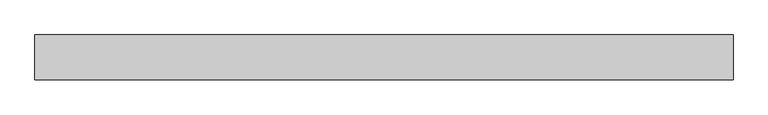
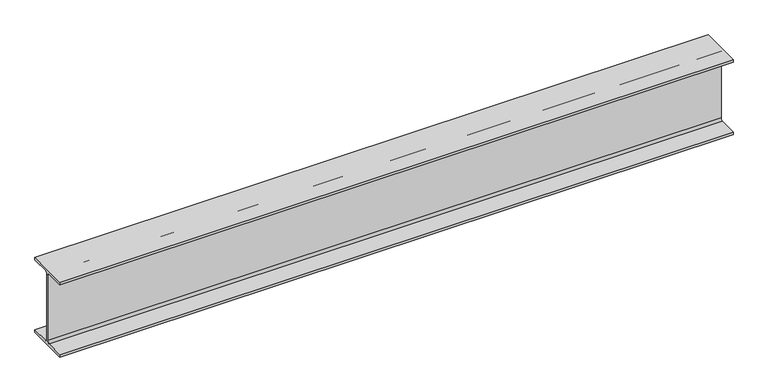
"""IFC4 building model written with IfcOpenShell, lengths in millimetres: beam geometry, Steel Beam_H-KSD3502 : H_SB_ASB_H-194x150x6x9."""

import ifcopenshell
import ifcopenshell.guid

model = None  # the IFC model being written
_history = None  # IfcOwnerHistory: only IFC2X3 demands one
_inside = {}  # id of a spatial element -> (the spatial element, [elements in it])
_under = {}  # id of a project, library or spatial element -> (it, [spatial elements below it])
_declared = {}  # id of a project -> (the project, [libraries it declares])
_typed = {}  # id of a type object -> (the type object, [elements of that type])
_made_of = {}  # id of a material, layer set ... -> (it, [elements and type objects made of it])


def new_model(schema):
    """Start an empty IFC model of exactly this schema.

    Asked for "IFC4X3", IfcOpenShell would pick the latest addendum, in which some entities
    have other attributes; the version numbers below select the first issue.
    IFC2X3 requires an IfcOwnerHistory on every rooted entity: one is made here for all.
    """
    global model, _history
    if schema == "IFC4X3":
        model = ifcopenshell.file(schema_version=(4, 3, 0, 0))
    else:
        model = ifcopenshell.file(schema=schema)
    _inside.clear()
    _under.clear()
    _declared.clear()
    _typed.clear()
    _made_of.clear()
    _history = None
    if model.schema == "IFC2X3":
        org = make("IfcOrganization", Name="unknown")
        user = make(
            "IfcPersonAndOrganization",
            ThePerson=make("IfcPerson", FamilyName="unknown"),
            TheOrganization=org,
        )
        app = make(
            "IfcApplication",
            ApplicationDeveloper=org,
            Version="unknown",
            ApplicationFullName="unknown",
            ApplicationIdentifier="unknown",
        )
        _history = make(
            "IfcOwnerHistory",
            OwningUser=user,
            OwningApplication=app,
            ChangeAction="ADDED",
            CreationDate=0,
        )
    return model


def make(cls, **values):
    """One entity of the class cls with the attributes given. An attribute that is None is left unset."""
    return model.create_entity(
        cls, **{name: value for name, value in values.items() if value is not None}
    )


def rooted(cls, **values):
    """An entity with a GlobalId (a new one), such as an element, a storey or a relation."""
    return make(cls, GlobalId=ifcopenshell.guid.new(), OwnerHistory=_history, **values)


def si_unit(unit_type, name, prefix=None):
    """IfcSIUnit, for example si_unit("LENGTHUNIT", "METRE", prefix="MILLI")."""
    return make("IfcSIUnit", UnitType=unit_type, Prefix=prefix, Name=name)


def assignment(units):
    """IfcUnitAssignment: the units of a project."""
    return None if units is None else make("IfcUnitAssignment", Units=units)


def point(xyz):
    """IfcCartesianPoint."""
    return None if xyz is None else make("IfcCartesianPoint", Coordinates=xyz)


def direction(xyz):
    """IfcDirection."""
    return None if xyz is None else make("IfcDirection", DirectionRatios=xyz)


def frame(location, z_axis=None, x_axis=None):
    """IfcAxis2Placement3D, a coordinate frame: its origin and axes. An axis left out is left unset."""
    return make(
        "IfcAxis2Placement3D",
        Location=point(location),
        Axis=direction(z_axis),
        RefDirection=direction(x_axis),
    )


def frame_2d(location, x_axis=None):
    """IfcAxis2Placement2D, a coordinate frame in the plane: its origin and x axis."""
    return make(
        "IfcAxis2Placement2D", Location=point(location), RefDirection=direction(x_axis)
    )


def origin():
    """The frame at (0, 0, 0) with its axes left unset."""
    return frame((0.0, 0.0, 0.0))


def place(relative_to, where):
    """IfcLocalPlacement: puts the frame where relative to a parent placement (None: the world)."""
    return make(
        "IfcLocalPlacement", PlacementRelTo=relative_to, RelativePlacement=where
    )


def context(
    kind, dimensions, precision=None, world=None, true_north=None, identifier=None
):
    """IfcGeometricRepresentationContext, for example the 3D "Model" context."""
    return make(
        "IfcGeometricRepresentationContext",
        ContextIdentifier=identifier,
        ContextType=kind,
        CoordinateSpaceDimension=dimensions,
        Precision=precision,
        WorldCoordinateSystem=world,
        TrueNorth=true_north,
    )


def project(units=None, contexts=None):
    """IfcProject with its units and contexts."""
    return rooted(
        "IfcProject",
        Name="project",
        RepresentationContexts=contexts,
        UnitsInContext=assignment(units),
    )


def spatial(cls, under=None, at=None, **own):
    """A site, building, storey or space (cls), placed at a placement, below another one or the project."""
    s = rooted(cls, ObjectPlacement=at, **own)
    if under is not None:
        _under.setdefault(under.id(), (under, []))[1].append(s)
    return s


def polyline(points):
    """IfcPolyline through the points."""
    return make("IfcPolyline", Points=[point(p) for p in points])


def circle_curve(where, radius):
    """IfcCircle in the frame where."""
    return make("IfcCircle", Position=where, Radius=radius)


def trimmed(basis, trim1, trim2, sense, master):
    """IfcTrimmedCurve: the piece of a basis curve between two trims."""
    return make(
        "IfcTrimmedCurve",
        BasisCurve=basis,
        Trim1=trim1,
        Trim2=trim2,
        SenseAgreement=sense,
        MasterRepresentation=master,
    )


def segment(curve, same_sense, transition):
    """IfcCompositeCurveSegment."""
    return make(
        "IfcCompositeCurveSegment",
        Transition=transition,
        SameSense=same_sense,
        ParentCurve=curve,
    )


def composite_curve(segments, self_intersect=None):
    """IfcCompositeCurve: segments joined end to end."""
    return make("IfcCompositeCurve", Segments=segments, SelfIntersect=self_intersect)


def outline(outer, holes=None, kind="AREA"):
    """IfcArbitraryClosedProfileDef: a profile drawn as a closed curve; with holes, ...WithVoids."""
    if holes is None:
        return make("IfcArbitraryClosedProfileDef", ProfileType=kind, OuterCurve=outer)
    return make(
        "IfcArbitraryProfileDefWithVoids",
        ProfileType=kind,
        OuterCurve=outer,
        InnerCurves=holes,
    )


def extrude(swept, where, along, depth):
    """IfcExtrudedAreaSolid: the profile swept, set in the frame where, extruded along a direction by depth."""
    return make(
        "IfcExtrudedAreaSolid",
        SweptArea=swept,
        Position=where,
        ExtrudedDirection=direction(along),
        Depth=depth,
    )


def shape(context_of_items, identifier, shape_type, items):
    """IfcShapeRepresentation: the items that make up one representation, for example the "Body"."""
    return make(
        "IfcShapeRepresentation",
        ContextOfItems=context_of_items,
        RepresentationIdentifier=identifier,
        RepresentationType=shape_type,
        Items=items,
    )


def source(mapping_origin, context_of_items, identifier, shape_type, items):
    """IfcRepresentationMap: a shape defined once, which mapped items show again and again."""
    return make(
        "IfcRepresentationMap",
        MappingOrigin=mapping_origin,
        MappedRepresentation=shape(context_of_items, identifier, shape_type, items),
    )


def transform(
    local_origin,
    x_axis=None,
    y_axis=None,
    z_axis=None,
    scale=None,
    scale2=None,
    scale3=None,
    uniform=True,
):
    """IfcCartesianTransformationOperator3D, or its non-uniform kind. x_axis, y_axis, z_axis: its Axis1, 2, 3."""
    if uniform:
        return make(
            "IfcCartesianTransformationOperator3D",
            Axis1=direction(x_axis),
            Axis2=direction(y_axis),
            LocalOrigin=point(local_origin),
            Scale=scale,
            Axis3=direction(z_axis),
        )
    return make(
        "IfcCartesianTransformationOperator3DnonUniform",
        Axis1=direction(x_axis),
        Axis2=direction(y_axis),
        LocalOrigin=point(local_origin),
        Scale=scale,
        Axis3=direction(z_axis),
        Scale2=scale2,
        Scale3=scale3,
    )


def mapped(mapping_source, mapping_target):
    """IfcMappedItem: shows the shape of a source again, moved by a transform."""
    return make(
        "IfcMappedItem", MappingSource=mapping_source, MappingTarget=mapping_target
    )


def made_of(thing, what):
    """Note that an element or type object is made of a material, layer set ...; save() writes the relation."""
    if what is not None:
        _made_of.setdefault(what.id(), (what, []))[1].append(thing)
    return thing


def element(
    cls,
    number,
    at=None,
    inside=None,
    cuts=None,
    type_object=None,
    material=None,
    context=None,
    identifier="Body",
    shape_type=None,
    held_by="IfcProductDefinitionShape",
    body=None,
    shapes=None,
    **own,
):
    """One element of the class cls, such as IfcWall. Its Tag is "e" and its number.

    at: its placement. inside: the storey or other place that contains it. cuts: it is an
    opening in that element (IfcRelVoidsElement). A single representation is given by context,
    identifier, shape_type and body (its items); several are given by shapes. held_by: the class
    of the entity that holds the representations. save() writes the other relations.
    """
    e = rooted(cls, Tag="e%d" % number, ObjectPlacement=at, **own)
    if body is not None:
        shapes = [shape(context, identifier, shape_type, body)]
    if shapes is not None:
        e.Representation = make(held_by, Representations=shapes)
    if inside is not None:
        _inside.setdefault(inside.id(), (inside, []))[1].append(e)
    if cuts is not None:
        rooted(
            "IfcRelVoidsElement", RelatingBuildingElement=cuts, RelatedOpeningElement=e
        )
    if type_object is not None:
        _typed.setdefault(type_object.id(), (type_object, []))[1].append(e)
    return made_of(e, material)


def aggregate(whole, parts):
    """IfcRelAggregates: a whole, such as a stair, and the parts it consists of."""
    return rooted("IfcRelAggregates", RelatingObject=whole, RelatedObjects=parts)


def save(model, path):
    """Write the relations noted so far, then the file.

    IfcRelAggregates (storeys below a building ...), IfcRelContainedInSpatialStructure (elements
    in a storey), IfcRelDefinesByType, IfcRelAssociatesMaterial and IfcRelDeclares: one each for
    every whole, place, type object, material and project.
    """
    for whole, parts in _under.values():
        aggregate(whole, parts)
    for where, things in _inside.values():
        rooted(
            "IfcRelContainedInSpatialStructure",
            RelatedElements=things,
            RelatingStructure=where,
        )
    for kind, things in _typed.values():
        rooted("IfcRelDefinesByType", RelatedObjects=things, RelatingType=kind)
    for what, things in _made_of.values():
        rooted("IfcRelAssociatesMaterial", RelatedObjects=things, RelatingMaterial=what)
    for by, libraries in _declared.values():
        rooted("IfcRelDeclares", RelatingContext=by, RelatedDefinitions=libraries)
    model.write(path)


def beam_c1192738(model_context):
    return source(origin(), model_context, "Body", "SweptSolid", [
        extrude(outline(composite_curve([segment(polyline([(82.5, -141.5), (82.5, -151.7), (-82.5, -151.7), (-82.5, -141.5), (-11.9, -141.5)]), True, "CONTINUOUS"), segment(trimmed(circle_curve(frame_2d((-11.9, -132.6)), 8.9), [point((-11.9, -141.5))], [point((-3.0, -132.6))], True, "CARTESIAN"), True, "CONTINUOUS"), segment(polyline([(-3.0, -132.6), (-3.0, 132.6)]), True, "CONTINUOUS"), segment(trimmed(circle_curve(frame_2d((-11.9, 132.6)), 8.9), [point((-3.0, 132.6))], [point((-11.9, 141.5))], True, "CARTESIAN"), True, "CONTINUOUS"), segment(polyline([(-11.9, 141.5), (-82.5, 141.5), (-82.5, 151.7), (82.5, 151.7), (82.5, 141.5), (11.9, 141.5)]), True, "CONTINUOUS"), segment(trimmed(circle_curve(frame_2d((11.9, 132.6)), 8.9), [point((11.9, 141.5))], [point((3.0, 132.6))], True, "CARTESIAN"), True, "CONTINUOUS"), segment(polyline([(3.0, 132.6), (3.0, -132.6)]), True, "CONTINUOUS"), segment(trimmed(circle_curve(frame_2d((11.9, -132.6)), 8.9), [point((3.0, -132.6))], [point((11.9, -141.5))], True, "CARTESIAN"), True, "CONTINUOUS"), segment(polyline([(11.9, -141.5), (82.5, -141.5)]), True, "CONTINUOUS")], self_intersect=False)), frame((-1265.0, 0.0, 0.0), z_axis=(1.0, 0.0, 0.0), x_axis=(0.0, 1.0, 0.0)), (0.0, 0.0, 1.0), 2578.0465428),
    ])


if __name__ == "__main__":
    model = new_model("IFC4")
    model_context = context("Model", 3, world=origin())
    ifc_project = project(units=[si_unit("LENGTHUNIT", "METRE", prefix="MILLI")], contexts=[model_context])
    site = spatial("IfcSite", under=ifc_project)
    building = spatial("IfcBuilding", under=site)
    placement = place(None, origin())
    beam_shape = beam_c1192738(model_context)
    element("IfcBeam", 1, ObjectType="Steel Beam_H-KSD3502 : H_SB_ASB_H-194x150x6x9", at=placement, inside=building, context=model_context, shape_type="MappedRepresentation", body=[
        mapped(beam_shape, transform((0.0, 0.0, 0.0), x_axis=(1.0, 0.0, 0.0), y_axis=(0.0, 1.0, 0.0), z_axis=(0.0, 0.0, 1.0))),
    ])
    save(model, "model.ifc")

# Revit data of these elements
# Type "Steel Beam_H-KSD3502 : H_SB_ASB_H-194x150x6x9"
#   Width = 15.0 cm
#   Web Thickness = 0.6 cm
#   Web Fillet = 1.3 cm
#   Warping Constant = 43316.0 cm⁶
#   Torsional Moment of Inertia = 8.622 cm⁴
#   Torsional Modulus = 1.0 cm³
#   Section Area = 39.01 cm²
#   Plastic Modulus weak axis = 104.0 cm³
#   Plastic Modulus strong axis = 309.0 cm³
#   Perimeter = 0.95 m²/m
#   Nominal Weight = 30.60 kgf/m
#   Moment of Inertia weak axis = 507.00 cm⁴
#   Moment of Inertia strong axis = 2690.00 cm⁴
#   Height = 19.4 cm
#   Flange Thickness = 0.9 cm
#   Elastic Modulus weak axis = 67.6 cm³
#   Elastic Modulus strong axis = 277.0 cm³
#   Centroid Vertical = 9.7 cm
#   Centroid Horizontal = 7.5 cm
#   Length [instance default] = 1.5240 m
#   Structural Material [instance default] = Steel, 45-345
#   Assembly Code = ""
# Element 1 (IfcBeam, "Steel Beam_H-KSD3502 : H_SB_ASB_H-194x150x6x9")
#   Structural Material = none
# Materials
#   "Steel, 45-345": class "Metal", colour RGB 189 187 185, transparency 0, Description = "Steel 345 MPa", Cost = 0
